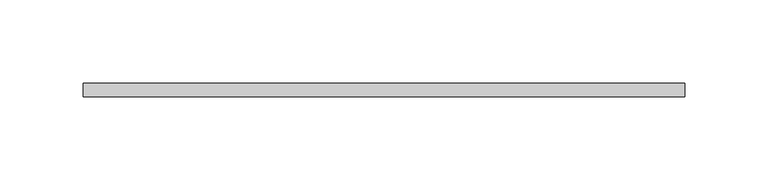
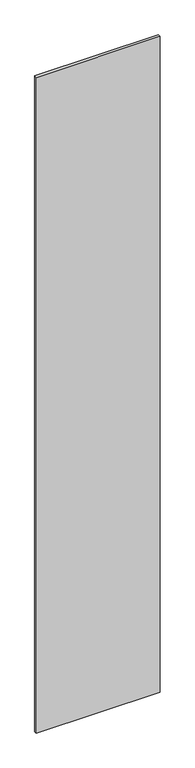
"""IFC4 building model written with IfcOpenShell, lengths in millimetres: proxy geometry, Panel:Panel:300402:Panel:300402 : Panel:Panel:300402:300124:Panel:300402:Panel:300402 : Panel:Panel:300402:300124 : Panel:Panel:300402:Panel:300402 : Panel:Panel:300402:300124:10 : Panel:Panel:300402:Panel:300402 : Panel:Panel:300402:300124:Panel:300402:Panel:300402 : Panel:Panel:300402:300124 : Panel:Panel:300402:Panel:300402 : Panel:Panel:300402:300124:300083."""

from ifc_helpers import new_model, si_unit, frame, origin, place, context, project, spatial, polyline, outline, extrude, source, transform, mapped, element, save


def generic_models_519c0b38(model_context):
    return source(origin(), model_context, "Body", "SweptSolid", [
        extrude(outline(polyline([(577805.9367239, -579076.8913841), (578166.2992239, -579076.8913841), (578166.2992239, -579084.8288841), (577805.9367239, -579084.8288841), (577805.9367239, -579076.8913841)])), frame((0.0, 0.0, 4118.0888261), z_axis=(0.0, 0.0, 1.0), x_axis=(1.0, 0.0, 0.0)), (0.0, 0.0, 1.0), 2016.0111739),
    ])


if __name__ == "__main__":
    model = new_model("IFC4")
    model_context = context("Model", 3, world=origin())
    ifc_project = project(units=[si_unit("LENGTHUNIT", "METRE", prefix="MILLI")], contexts=[model_context])
    site = spatial("IfcSite", under=ifc_project)
    building = spatial("IfcBuilding", under=site)
    placement = place(None, origin())
    generic_models_shape = generic_models_519c0b38(model_context)
    element("IfcBuildingElementProxy", 1, Name="Panel:Panel:300402:Panel:300402 : Panel:Panel:300402:300124:Panel:300402:Panel:300402 : Panel:Panel:300402:300124 : Panel:Panel:300402:Panel:300402 : Panel:Panel:300402:300124:10 : Panel:Panel:300402:Panel:300402 : Panel:Panel:300402:300124:Panel:300402:Panel:300402 : Panel:Panel:300402:300124 : Panel:Panel:300402:Panel:300402 : Panel:Panel:300402:300124:300083", ObjectType="Panel:Panel:300402:Panel:300402 : Panel:Panel:300402:300124:Panel:300402:Panel:300402 : Panel:Panel:300402:300124 : Panel:Panel:300402:Panel:300402 : Panel:Panel:300402:300124:10 : Panel:Panel:300402:Panel:300402 : Panel:Panel:300402:300124:Panel:300402:Panel:300402 : Panel:Panel:300402:300124 : Panel:Panel:300402:Panel:300402 : Panel:Panel:300402:300124:300083", at=placement, inside=building, context=model_context, shape_type="MappedRepresentation", body=[
        mapped(generic_models_shape, transform((0.0, 0.0, 0.0), x_axis=(1.0, 0.0, 0.0), y_axis=(0.0, 1.0, 0.0), z_axis=(0.0, 0.0, 1.0))),
    ])
    save(model, "model.ifc")

# Revit data of these elements
# Type "Panel:Panel:300402:Panel:300402 : Panel:Panel:300402:300124:Panel:300402:Panel:300402 : Panel:Panel:300402:300124 : Panel:Panel:300402:Panel:300402 : Panel:Panel:300402:300124:10 : Panel:Panel:300402:Panel:300402 : Panel:Panel:300402:300124:Panel:300402:Panel:300402 : Panel:Panel:300402:300124 : Panel:Panel:300402:Panel:300402 : Panel:Panel:300402:300124:300083"
#   NameOverride = "Panel:Panel:300402:Panel:300402 : Panel:Panel:300402:300124:Panel:300402:Panel:300402 : Panel:Panel:300402:300124 : Panel:Panel:300402:Panel:300402 : Panel:Panel:300402:300124:300083"
#   ObjectTypeOverride = "Panel:300402:Panel:300402 : Panel:Panel:300402:300124 : Panel:Panel:300402:Panel:300402 : Panel:Panel:300402:300124"
#   Reference = "Panel"
#   Tag = "300083"
# Element 1 (IfcBuildingElementProxy, "Panel:Panel:300402:Panel:300402 : Panel:Panel:300402:300124:Panel:300402:Panel:300402 : Panel:Panel:300402:300124 : Panel:Panel:300402:Panel:300402 : Panel:Panel:300402:300124:10 : Panel:Panel:300402:Panel:300402 : Panel:Panel:300402:300124:Panel:300402:Panel:300402 : Panel:Panel:300402:300124 : Panel:Panel:300402:Panel:300402 : Panel:Panel:300402:300124:300083")
#   Materials on its faces: "5/16\" THICK STONEWOOD RESIN PANELS - EXPOSED FASTENERS"
# Materials
#   "5/16\" THICK STONEWOOD RESIN PANELS - EXPOSED FASTENERS": class "Unassigned", colour RGB 64 64 64, transparency 0, Keynote = "M07420000.01", Cost = 0
